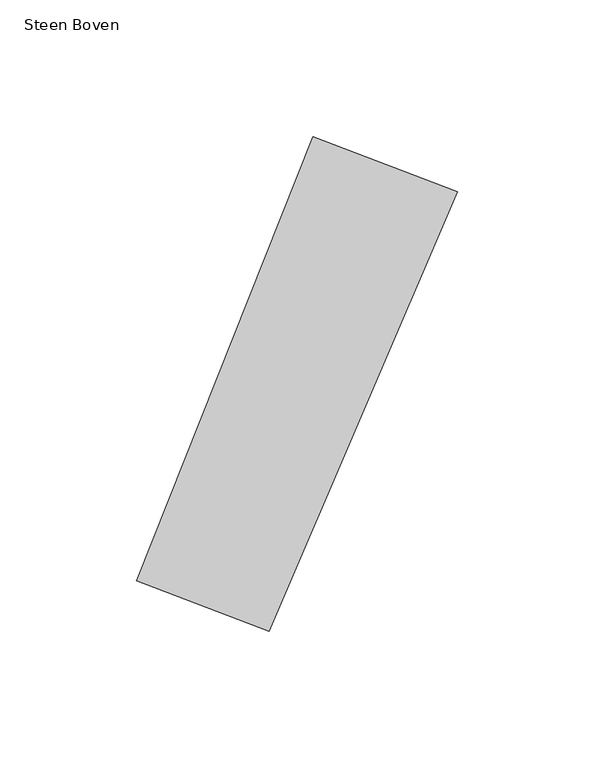
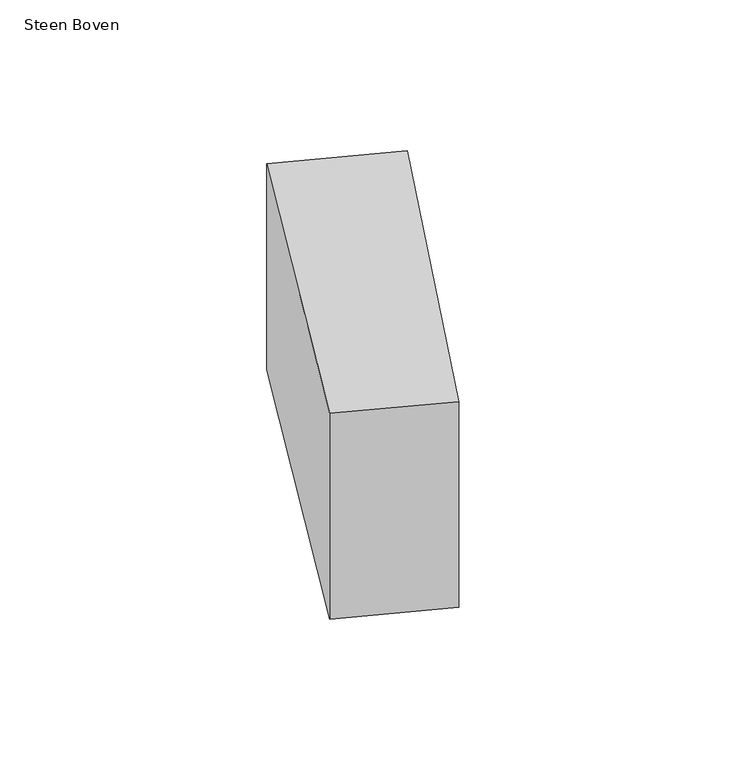
"""IFC4 building model written with IfcOpenShell, lengths in millimetres: proxy geometry, 00_GMA_steen_versie_4 : Steen Boven."""

from ifc_helpers import new_model, si_unit, origin, origin_with_axes, place, context, project, spatial, polyline, outline, extrude, source, transform, mapped, element, save


def steen_boven_08d21662(model_context):
    return source(origin(), model_context, "Body", "SweptSolid", [
        extrude(outline(polyline([(136.4236357, 153.1478915), (67.3165894, -7.7853757), (18.7549708, 10.8090642), (83.5026061, 173.4080924), (136.4236357, 153.1478915)])), origin_with_axes(), (0.0, 0.0, 1.0), 100.0),
    ])


if __name__ == "__main__":
    model = new_model("IFC4")
    model_context = context("Model", 3, world=origin())
    ifc_project = project(units=[si_unit("LENGTHUNIT", "METRE", prefix="MILLI")], contexts=[model_context])
    site = spatial("IfcSite", under=ifc_project)
    building = spatial("IfcBuilding", under=site)
    placement = place(None, origin())
    steen_boven_shape = steen_boven_08d21662(model_context)
    element("IfcBuildingElementProxy", 1, Name="00_GMA_steen_versie_4 : Steen Boven", ObjectType="00_GMA_steen_versie_4 : Steen Boven", at=placement, inside=building, context=model_context, shape_type="MappedRepresentation", body=[
        mapped(steen_boven_shape, transform((0.0, 0.0, 0.0), x_axis=(1.0, 0.0, 0.0), y_axis=(0.0, 1.0, 0.0), z_axis=(0.0, 0.0, 1.0))),
    ])
    save(model, "model.ifc")

# Revit data of these elements
# Type "00_GMA_steen_versie_4 : Steen Boven"
#   StootVoegHalfBoven [instance default] = 5 mm
#   StootVoegHalf [instance default] = 5 mm
#   StootVoegBreedteOnder = 10 mm
#   StootVoegBreedteBoven = 10 mm
#   Steendikte = 100 mm
#   LintVoegOnderHalf = 5 mm
#   LintVoegOnder = 10 mm
#   LintVoegBovenHalf = 0 mm
#   LintVoegBoven = 0 mm
#   materiaal = none
#   MateriaalVoeg = none
#   Default Elevation = 0
